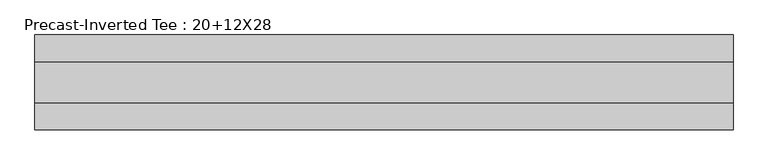
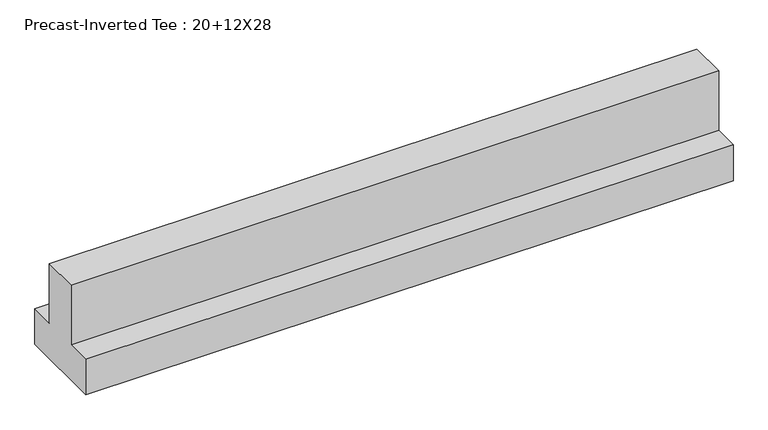
"""IFC4 building model written with IfcOpenShell, lengths in millimetres: beam geometry, Precast-Inverted Tee : 20+12X28."""

from ifc_helpers import new_model, si_unit, frame, origin, place, context, project, spatial, polyline, outline, extrude, source, transform, mapped, element, save


def precast_inverted_tee_20_12x28_77df7164(model_context):
    return source(origin(), model_context, "Body", "SweptSolid", [
        extrude(outline(polyline([(-355.6, -406.4), (-355.6, -101.6), (-152.4, -101.6), (-152.4, 406.4), (152.4, 406.4), (152.4, -101.6), (355.6, -101.6), (355.6, -406.4), (-355.6, -406.4)])), frame((-2728.5280327, 0.0, 0.0), z_axis=(1.0, 0.0, 0.0), x_axis=(0.0, 1.0, 0.0)), (0.0, 0.0, 1.0), 5228.4560654),
    ])


if __name__ == "__main__":
    model = new_model("IFC4")
    model_context = context("Model", 3, world=origin())
    ifc_project = project(units=[si_unit("LENGTHUNIT", "METRE", prefix="MILLI")], contexts=[model_context])
    site = spatial("IfcSite", under=ifc_project)
    building = spatial("IfcBuilding", under=site)
    placement = place(None, origin())
    precast_inverted_tee_20_12x28_shape = precast_inverted_tee_20_12x28_77df7164(model_context)
    element("IfcBeam", 1, ObjectType="Precast-Inverted Tee : 20+12X28", at=placement, inside=building, context=model_context, shape_type="MappedRepresentation", body=[
        mapped(precast_inverted_tee_20_12x28_shape, transform((0.0, 0.0, 0.0), x_axis=(1.0, 0.0, 0.0), y_axis=(0.0, 1.0, 0.0), z_axis=(0.0, 0.0, 1.0))),
    ])
    save(model, "model.ifc")

# Revit data of these elements
# Type "Precast-Inverted Tee : 20+12X28"
#   Assembly Code = "B10"
#   Seat = 0' - 8"
#   Length [instance default] = 5' - 0"
#   b = 2' - 4"
#   h = 2' - 8"
#   h1 = 1' - 8"
#   Structural Material [instance default] = Concrete - Precast Concrete - Normal Weight Concrete - 5 ksi
# Element 1 (IfcBeam, "Precast-Inverted Tee : 20+12X28")
#   Length = 17' - 5.84473"
#   Materials on its faces: "Concrete - Precast Concrete - Normal Weight Concrete - 5 ksi"
# Materials
#   "Concrete - Precast Concrete - Normal Weight Concrete - 5 ksi": class "Concrete", colour RGB 198 187 187, transparency 0, Cost = 0
